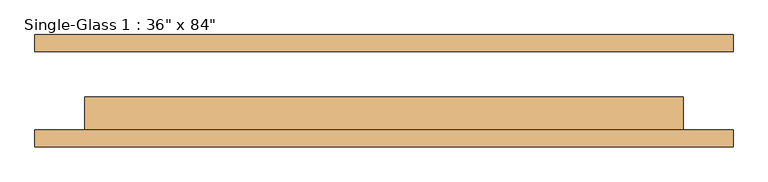
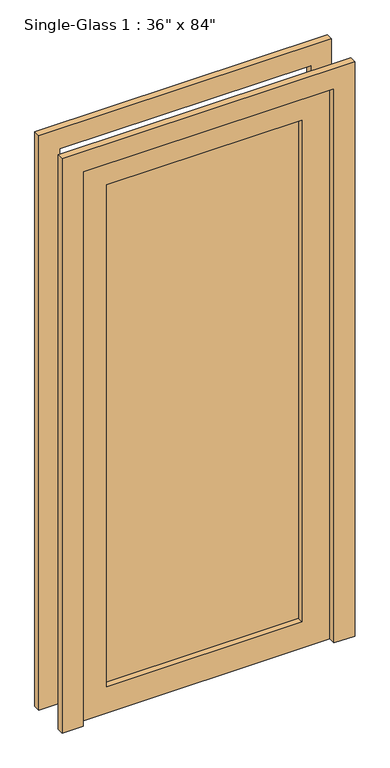
"""IFC4 building model written with IfcOpenShell, lengths in millimetres: door geometry."""

from ifc_helpers import new_model, si_unit, frame, origin, place, context, project, spatial, polyline, outline, extrude, source, transform, mapped, element, save


def door_84b54e47(model_context):
    return source(origin(), model_context, "Body", "SweptSolid", [
        extrude(outline(polyline([(2133.6, 457.2), (0.0, 457.2), (0.0, 533.4), (2209.8, 533.4), (2209.8, -533.4), (0.0, -533.4), (0.0, -457.2), (2133.6, -457.2), (2133.6, 457.2)])), frame((0.0, 60.325, 0.0), z_axis=(0.0, 1.0, 0.0), x_axis=(0.0, 0.0, 1.0)), (0.0, 0.0, 1.0), 25.4),
        extrude(outline(polyline([(2133.6, 457.2), (0.0, 457.2), (0.0, 533.4), (2209.8, 533.4), (2209.8, -533.4), (0.0, -533.4), (0.0, -457.2), (2133.6, -457.2), (2133.6, 457.2)])), frame((0.0, -85.725, 0.0), z_axis=(0.0, 1.0, 0.0), x_axis=(0.0, 0.0, 1.0)), (0.0, 0.0, 1.0), 25.4),
        extrude(outline(polyline([(355.6, -31.75), (355.6, -38.1), (-355.6, -38.1), (-355.6, -31.75), (355.6, -31.75)])), frame((0.0, 0.0, 101.6), z_axis=(0.0, 0.0, 1.0), x_axis=(1.0, 0.0, 0.0)), (0.0, 0.0, 1.0), 1930.4),
        extrude(outline(polyline([(2133.6, 457.2), (2133.6, -457.2), (0.0, -457.2), (0.0, 457.2), (2133.6, 457.2)]), holes=[polyline([(2032.0, -355.6), (2032.0, 355.6), (101.6, 355.6), (101.6, -355.6), (2032.0, -355.6)])]), frame((0.0, -60.325, 0.0), z_axis=(0.0, 1.0, 0.0), x_axis=(0.0, 0.0, 1.0)), (0.0, 0.0, 1.0), 50.8),
    ])


if __name__ == "__main__":
    model = new_model("IFC4")
    model_context = context("Model", 3, world=origin())
    ifc_project = project(units=[si_unit("LENGTHUNIT", "METRE", prefix="MILLI")], contexts=[model_context])
    site = spatial("IfcSite", under=ifc_project)
    building = spatial("IfcBuilding", under=site)
    placement = place(None, origin())
    door_shape = door_84b54e47(model_context)
    element("IfcDoor", 1, ObjectType="Single-Glass 1 : 36\" x 84\"", at=placement, inside=building, context=model_context, shape_type="MappedRepresentation", body=[
        mapped(door_shape, transform((0.0, 0.0, 0.0), x_axis=(1.0, 0.0, 0.0), y_axis=(0.0, 1.0, 0.0), z_axis=(0.0, 0.0, 1.0))),
    ])
    save(model, "model.ifc")

# Revit data of these elements
# Type "Single-Glass 1 : 36\" x 84\""
#   Type Mark = "20"
#   Construction Type Id = "MDOOR"
#   Assembly Code = "C1020"
#   Analytic Construction = "Metal"
#   Thickness = 0' - 2"
#   Heat Transfer Coefficient (U) = 3.7021 W/(m²·K)
#   Height = 7' - 0"
#   Rail Width - Base = 0' - 4"
#   Rail Width - Top = 0' - 4"
#   Stile Width - Hinge = 0' - 4"
#   Stile Width - Latch = 0' - 4"
#   Trim Projection Ext = 0' - 1"
#   Trim Projection Int = 0' - 1"
#   Trim Width = 0' - 3"
#   Width = 3' - 0"
#   Door Material = Aluminum
#   Frame Material = Aluminum
#   Visual Light Transmittance = 0
#   Solar Heat Gain Coefficient = 0
#   Function = (empty or 0)
#   Wall Closure = (empty or 0)
# Element 1 (IfcDoor, "Single-Glass 1 : 36\" x 84\"")
#   Materials on its faces: "Aluminum", "Glass"
# Materials
#   "Aluminum": class "Metal", colour RGB 226 226 226, transparency 0, Description = "Aluminum 6061", Cost = 0
#   "Glass": class "Glass", colour RGB 142 168 196, transparency 0.75, Description = "Soda Lime Glass", Cost = 0
